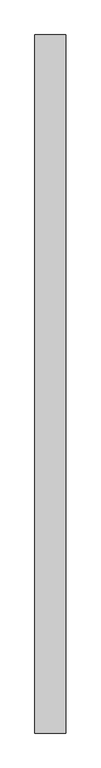
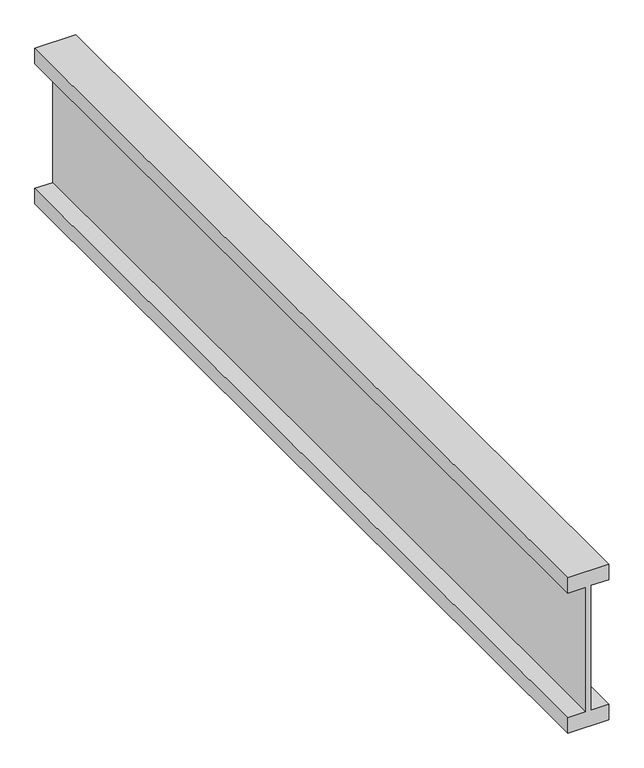
"""IFC4 building model written with IfcOpenShell, lengths in millimetres: proxy geometry, Framing 5:Framing 17515:302427 : Framing 5:Framing 17515:302427."""

from ifc_helpers import new_model, si_unit, frame, origin, place, context, project, spatial, polyline, outline, extrude, source, transform, mapped, element, save


def generic_models_d18cc510(model_context):
    return source(origin(), model_context, "Body", "SweptSolid", [
        extrude(outline(polyline([(40077.771, 12428.011296), (40077.771, 12466.905046), (39792.021, 12466.905046), (39792.021, 12428.011296), (39757.096, 12428.011296), (39757.096, 12516.911296), (39792.021, 12516.911296), (39792.021, 12478.017546), (40077.771, 12478.017546), (40077.771, 12516.911296), (40112.696, 12516.911296), (40112.696, 12428.011296), (40077.771, 12428.011296)])), frame((0.0, -3469.6166527, 0.0), z_axis=(0.0, 1.0, 0.0), x_axis=(0.0, 0.0, 1.0)), (0.0, 0.0, 1.0), 2000.0),
    ])


if __name__ == "__main__":
    model = new_model("IFC4")
    model_context = context("Model", 3, world=origin())
    ifc_project = project(units=[si_unit("LENGTHUNIT", "METRE", prefix="MILLI")], contexts=[model_context])
    site = spatial("IfcSite", under=ifc_project)
    building = spatial("IfcBuilding", under=site)
    placement = place(None, origin())
    generic_models_shape = generic_models_d18cc510(model_context)
    element("IfcBuildingElementProxy", 1, Name="Framing 5:Framing 17515:302427 : Framing 5:Framing 17515:302427", ObjectType="Framing 5:Framing 17515:302427 : Framing 5:Framing 17515:302427", at=placement, inside=building, context=model_context, shape_type="MappedRepresentation", body=[
        mapped(generic_models_shape, transform((0.0, 0.0, 0.0), x_axis=(1.0, 0.0, 0.0), y_axis=(0.0, 1.0, 0.0), z_axis=(0.0, 0.0, 1.0))),
    ])
    save(model, "model.ifc")

# Revit data of these elements
# Type "Framing 5:Framing 17515:302427 : Framing 5:Framing 17515:302427"
#   NameOverride = "Framing 5:Framing 17515:302427"
#   ObjectTypeOverride = "Framing 5:Framing 17515"
#   Reference = "Framing 17515"
#   Category = "Generic Models"
#   Tag = "302427"
# Element 1 (IfcBuildingElementProxy, "Framing 5:Framing 17515:302427 : Framing 5:Framing 17515:302427")
#   Materials on its faces: "WOOD FRAMING (SEE STRUCT DWGS)"
# Materials
#   "WOOD FRAMING (SEE STRUCT DWGS)": class "Unassigned", colour RGB 224 188 168, transparency 0, Cost = 0
